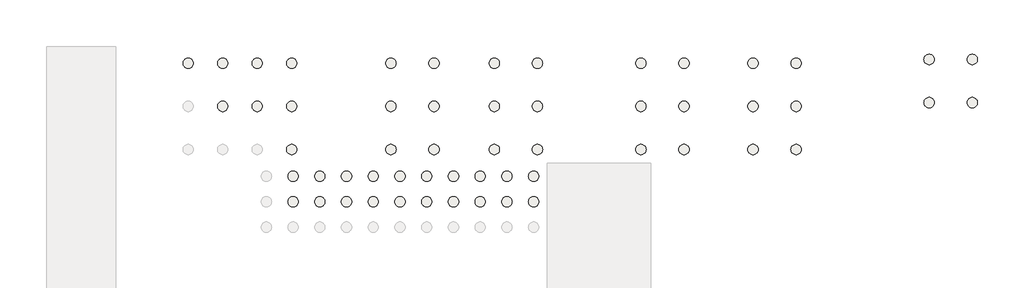
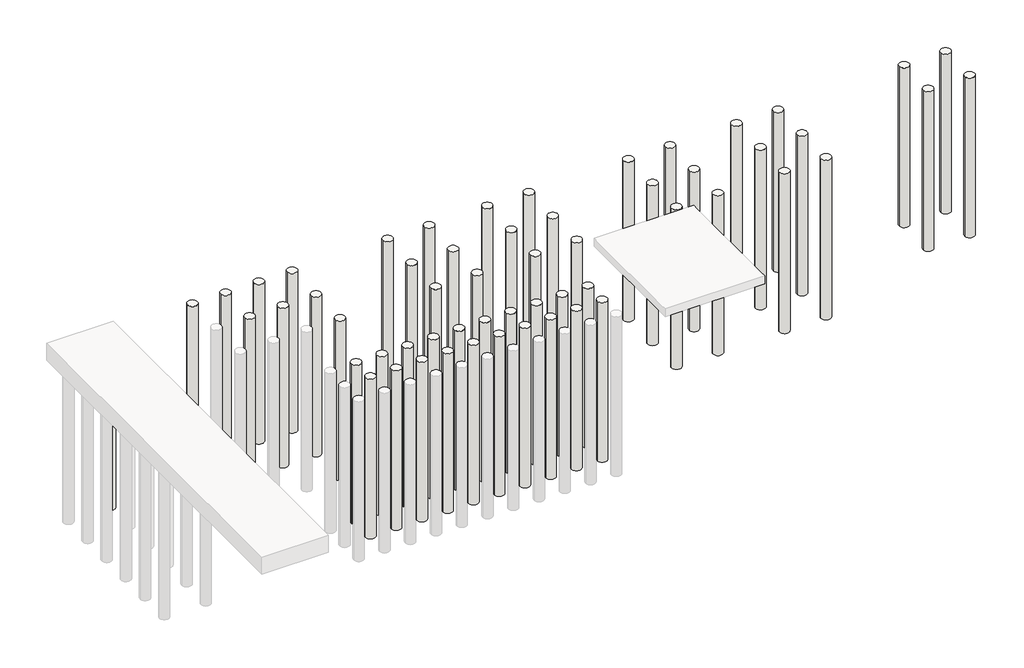
# One storey, part 3 of 3: 57 slabs.
"""IFC4 building model written with IfcOpenShell, lengths in millimetres."""

import ifcopenshell
import ifcopenshell.guid

model = None  # the IFC model being written
_history = None  # IfcOwnerHistory: only IFC2X3 demands one
_inside = {}  # id of a spatial element -> (the spatial element, [elements in it])
_under = {}  # id of a project, library or spatial element -> (it, [spatial elements below it])
_declared = {}  # id of a project -> (the project, [libraries it declares])
_typed = {}  # id of a type object -> (the type object, [elements of that type])
_made_of = {}  # id of a material, layer set ... -> (it, [elements and type objects made of it])


def new_model(schema):
    """Start an empty IFC model of exactly this schema.

    Asked for "IFC4X3", IfcOpenShell would pick the latest addendum, in which some entities
    have other attributes; the version numbers below select the first issue.
    IFC2X3 requires an IfcOwnerHistory on every rooted entity: one is made here for all.
    """
    global model, _history
    if schema == "IFC4X3":
        model = ifcopenshell.file(schema_version=(4, 3, 0, 0))
    else:
        model = ifcopenshell.file(schema=schema)
    _inside.clear()
    _under.clear()
    _declared.clear()
    _typed.clear()
    _made_of.clear()
    _history = None
    if model.schema == "IFC2X3":
        org = make("IfcOrganization", Name="unknown")
        user = make(
            "IfcPersonAndOrganization",
            ThePerson=make("IfcPerson", FamilyName="unknown"),
            TheOrganization=org,
        )
        app = make(
            "IfcApplication",
            ApplicationDeveloper=org,
            Version="unknown",
            ApplicationFullName="unknown",
            ApplicationIdentifier="unknown",
        )
        _history = make(
            "IfcOwnerHistory",
            OwningUser=user,
            OwningApplication=app,
            ChangeAction="ADDED",
            CreationDate=0,
        )
    return model


def make(cls, **values):
    """One entity of the class cls with the attributes given. An attribute that is None is left unset."""
    return model.create_entity(
        cls, **{name: value for name, value in values.items() if value is not None}
    )


def rooted(cls, **values):
    """An entity with a GlobalId (a new one), such as an element, a storey or a relation."""
    return make(cls, GlobalId=ifcopenshell.guid.new(), OwnerHistory=_history, **values)


def si_unit(unit_type, name, prefix=None):
    """IfcSIUnit, for example si_unit("LENGTHUNIT", "METRE", prefix="MILLI")."""
    return make("IfcSIUnit", UnitType=unit_type, Prefix=prefix, Name=name)


def assignment(units):
    """IfcUnitAssignment: the units of a project."""
    return None if units is None else make("IfcUnitAssignment", Units=units)


def point(xyz):
    """IfcCartesianPoint."""
    return None if xyz is None else make("IfcCartesianPoint", Coordinates=xyz)


def direction(xyz):
    """IfcDirection."""
    return None if xyz is None else make("IfcDirection", DirectionRatios=xyz)


def frame(location, z_axis=None, x_axis=None):
    """IfcAxis2Placement3D, a coordinate frame: its origin and axes. An axis left out is left unset."""
    return make(
        "IfcAxis2Placement3D",
        Location=point(location),
        Axis=direction(z_axis),
        RefDirection=direction(x_axis),
    )


def frame_2d(location, x_axis=None):
    """IfcAxis2Placement2D, a coordinate frame in the plane: its origin and x axis."""
    return make(
        "IfcAxis2Placement2D", Location=point(location), RefDirection=direction(x_axis)
    )


def origin():
    """The frame at (0, 0, 0) with its axes left unset."""
    return frame((0.0, 0.0, 0.0))


def place(relative_to, where):
    """IfcLocalPlacement: puts the frame where relative to a parent placement (None: the world)."""
    return make(
        "IfcLocalPlacement", PlacementRelTo=relative_to, RelativePlacement=where
    )


def context(
    kind, dimensions, precision=None, world=None, true_north=None, identifier=None
):
    """IfcGeometricRepresentationContext, for example the 3D "Model" context."""
    return make(
        "IfcGeometricRepresentationContext",
        ContextIdentifier=identifier,
        ContextType=kind,
        CoordinateSpaceDimension=dimensions,
        Precision=precision,
        WorldCoordinateSystem=world,
        TrueNorth=true_north,
    )


def project(units=None, contexts=None):
    """IfcProject with its units and contexts."""
    return rooted(
        "IfcProject",
        Name="project",
        RepresentationContexts=contexts,
        UnitsInContext=assignment(units),
    )


def spatial(cls, under=None, at=None, **own):
    """A site, building, storey or space (cls), placed at a placement, below another one or the project."""
    s = rooted(cls, ObjectPlacement=at, **own)
    if under is not None:
        _under.setdefault(under.id(), (under, []))[1].append(s)
    return s


def circle_curve(where, radius):
    """IfcCircle in the frame where."""
    return make("IfcCircle", Position=where, Radius=radius)


def trimmed(basis, trim1, trim2, sense, master):
    """IfcTrimmedCurve: the piece of a basis curve between two trims."""
    return make(
        "IfcTrimmedCurve",
        BasisCurve=basis,
        Trim1=trim1,
        Trim2=trim2,
        SenseAgreement=sense,
        MasterRepresentation=master,
    )


def segment(curve, same_sense, transition):
    """IfcCompositeCurveSegment."""
    return make(
        "IfcCompositeCurveSegment",
        Transition=transition,
        SameSense=same_sense,
        ParentCurve=curve,
    )


def composite_curve(segments, self_intersect=None):
    """IfcCompositeCurve: segments joined end to end."""
    return make("IfcCompositeCurve", Segments=segments, SelfIntersect=self_intersect)


def outline(outer, holes=None, kind="AREA"):
    """IfcArbitraryClosedProfileDef: a profile drawn as a closed curve; with holes, ...WithVoids."""
    if holes is None:
        return make("IfcArbitraryClosedProfileDef", ProfileType=kind, OuterCurve=outer)
    return make(
        "IfcArbitraryProfileDefWithVoids",
        ProfileType=kind,
        OuterCurve=outer,
        InnerCurves=holes,
    )


def extrude(swept, where, along, depth):
    """IfcExtrudedAreaSolid: the profile swept, set in the frame where, extruded along a direction by depth."""
    return make(
        "IfcExtrudedAreaSolid",
        SweptArea=swept,
        Position=where,
        ExtrudedDirection=direction(along),
        Depth=depth,
    )


def shape(context_of_items, identifier, shape_type, items):
    """IfcShapeRepresentation: the items that make up one representation, for example the "Body"."""
    return make(
        "IfcShapeRepresentation",
        ContextOfItems=context_of_items,
        RepresentationIdentifier=identifier,
        RepresentationType=shape_type,
        Items=items,
    )


def made_of(thing, what):
    """Note that an element or type object is made of a material, layer set ...; save() writes the relation."""
    if what is not None:
        _made_of.setdefault(what.id(), (what, []))[1].append(thing)
    return thing


def element(
    cls,
    number,
    at=None,
    inside=None,
    cuts=None,
    type_object=None,
    material=None,
    context=None,
    identifier="Body",
    shape_type=None,
    held_by="IfcProductDefinitionShape",
    body=None,
    shapes=None,
    **own,
):
    """One element of the class cls, such as IfcWall. Its Tag is "e" and its number.

    at: its placement. inside: the storey or other place that contains it. cuts: it is an
    opening in that element (IfcRelVoidsElement). A single representation is given by context,
    identifier, shape_type and body (its items); several are given by shapes. held_by: the class
    of the entity that holds the representations. save() writes the other relations.
    """
    e = rooted(cls, Tag="e%d" % number, ObjectPlacement=at, **own)
    if body is not None:
        shapes = [shape(context, identifier, shape_type, body)]
    if shapes is not None:
        e.Representation = make(held_by, Representations=shapes)
    if inside is not None:
        _inside.setdefault(inside.id(), (inside, []))[1].append(e)
    if cuts is not None:
        rooted(
            "IfcRelVoidsElement", RelatingBuildingElement=cuts, RelatedOpeningElement=e
        )
    if type_object is not None:
        _typed.setdefault(type_object.id(), (type_object, []))[1].append(e)
    return made_of(e, material)


def aggregate(whole, parts):
    """IfcRelAggregates: a whole, such as a stair, and the parts it consists of."""
    return rooted("IfcRelAggregates", RelatingObject=whole, RelatedObjects=parts)


def save(model, path):
    """Write the relations noted so far, then the file.

    IfcRelAggregates (storeys below a building ...), IfcRelContainedInSpatialStructure (elements
    in a storey), IfcRelDefinesByType, IfcRelAssociatesMaterial and IfcRelDeclares: one each for
    every whole, place, type object, material and project.
    """
    for whole, parts in _under.values():
        aggregate(whole, parts)
    for where, things in _inside.values():
        rooted(
            "IfcRelContainedInSpatialStructure",
            RelatedElements=things,
            RelatingStructure=where,
        )
    for kind, things in _typed.values():
        rooted("IfcRelDefinesByType", RelatedObjects=things, RelatingType=kind)
    for what, things in _made_of.values():
        rooted("IfcRelAssociatesMaterial", RelatedObjects=things, RelatingMaterial=what)
    for by, libraries in _declared.values():
        rooted("IfcRelDeclares", RelatingContext=by, RelatedDefinitions=libraries)
    model.write(path)


model = new_model("IFC4")

# Units and contexts
model_context = context("Model", 3, world=origin())
ifc_project = project(units=[si_unit("LENGTHUNIT", "METRE", prefix="MILLI")], contexts=[model_context])

# Site, building, storey
site = spatial("IfcSite", under=ifc_project)
building = spatial("IfcBuilding", under=site)
storey = spatial("IfcBuildingStorey", under=building, Name="B.O.F(FDN)", Elevation=-2500.0279945)

# Slabs
placement = place(None, origin())
element("IfcSlab", 1, ObjectType="Pile : H_SF_API_Steel Pile D508x12t_L10m", at=placement, inside=storey, context=model_context, shape_type="SweptSolid", body=[
    extrude(outline(composite_curve([segment(trimmed(circle_curve(frame_2d((1035.0, 40249.5208589)), 300.0), [point((1335.0, 40249.5208589))], [point((735.0, 40249.5208589))], False, "CARTESIAN"), True, "CONTINUOUS"), segment(trimmed(circle_curve(frame_2d((1035.0, 40249.5208589)), 300.0), [point((735.0, 40249.5208589))], [point((1335.0, 40249.5208589))], False, "CARTESIAN"), True, "CONTINUOUS")], self_intersect=False)), frame((0.0, 0.0, -13500.0279945), z_axis=(0.0, 0.0, 1.0), x_axis=(1.0, 0.0, 0.0)), (0.0, 0.0, 1.0), 10150.0),
])
element("IfcSlab", 2, ObjectType="Pile : H_SF_API_Steel Pile D508x12t_L10m", at=placement, inside=storey, context=model_context, shape_type="SweptSolid", body=[
    extrude(outline(composite_curve([segment(trimmed(circle_curve(frame_2d((51465.0, 37969.5208589)), 300.0), [point((51765.0, 37969.5208589))], [point((51165.0, 37969.5208589))], False, "CARTESIAN"), True, "CONTINUOUS"), segment(trimmed(circle_curve(frame_2d((51465.0, 37969.5208589)), 300.0), [point((51165.0, 37969.5208589))], [point((51765.0, 37969.5208589))], False, "CARTESIAN"), True, "CONTINUOUS")], self_intersect=False)), frame((0.0, 0.0, -12400.0279945), z_axis=(0.0, 0.0, 1.0), x_axis=(1.0, 0.0, 0.0)), (0.0, 0.0, 1.0), 10150.0),
])
element("IfcSlab", 3, ObjectType="Pile : H_SF_API_Steel Pile D508x12t_L10m", at=placement, inside=storey, context=model_context, shape_type="SweptSolid", body=[
    extrude(outline(composite_curve([segment(trimmed(circle_curve(frame_2d((48965.0, 37969.5208589)), 300.0), [point((48665.0, 37969.5208589))], [point((49265.0, 37969.5208589))], False, "CARTESIAN"), True, "CONTINUOUS"), segment(trimmed(circle_curve(frame_2d((48965.0, 37969.5208589)), 300.0), [point((49265.0, 37969.5208589))], [point((48665.0, 37969.5208589))], False, "CARTESIAN"), True, "CONTINUOUS")], self_intersect=False)), frame((0.0, 0.0, -12400.0279945), z_axis=(0.0, 0.0, 1.0), x_axis=(1.0, 0.0, 0.0)), (0.0, 0.0, 1.0), 10150.0),
])
element("IfcSlab", 4, ObjectType="Pile : H_SF_API_Steel Pile D508x12t_L10m", at=placement, inside=storey, context=model_context, shape_type="SweptSolid", body=[
    extrude(outline(composite_curve([segment(trimmed(circle_curve(frame_2d((51465.0, 40469.5208589)), 300.0), [point((51765.0, 40469.5208589))], [point((51165.0, 40469.5208589))], False, "CARTESIAN"), True, "CONTINUOUS"), segment(trimmed(circle_curve(frame_2d((51465.0, 40469.5208589)), 300.0), [point((51165.0, 40469.5208589))], [point((51765.0, 40469.5208589))], False, "CARTESIAN"), True, "CONTINUOUS")], self_intersect=False)), frame((0.0, 0.0, -12400.0279945), z_axis=(0.0, 0.0, 1.0), x_axis=(1.0, 0.0, 0.0)), (0.0, 0.0, 1.0), 10150.0),
])
element("IfcSlab", 5, ObjectType="Pile : H_SF_API_Steel Pile D508x12t_L10m", at=placement, inside=storey, context=model_context, shape_type="SweptSolid", body=[
    extrude(outline(composite_curve([segment(trimmed(circle_curve(frame_2d((48965.0, 40469.5208589)), 300.0), [point((48665.0, 40469.5208589))], [point((49265.0, 40469.5208589))], False, "CARTESIAN"), True, "CONTINUOUS"), segment(trimmed(circle_curve(frame_2d((48965.0, 40469.5208589)), 300.0), [point((49265.0, 40469.5208589))], [point((48665.0, 40469.5208589))], False, "CARTESIAN"), True, "CONTINUOUS")], self_intersect=False)), frame((0.0, 0.0, -12400.0279945), z_axis=(0.0, 0.0, 1.0), x_axis=(1.0, 0.0, 0.0)), (0.0, 0.0, 1.0), 10150.0),
])
element("IfcSlab", 6, ObjectType="Pile : H_SF_API_Steel Pile D508x12t_L10m", at=placement, inside=storey, context=model_context, shape_type="SweptSolid", body=[
    extrude(outline(composite_curve([segment(trimmed(circle_curve(frame_2d((6000.0, 40249.5208589)), 300.0), [point((5700.0, 40249.5208589))], [point((6300.0, 40249.5208589))], False, "CARTESIAN"), True, "CONTINUOUS"), segment(trimmed(circle_curve(frame_2d((6000.0, 40249.5208589)), 300.0), [point((6300.0, 40249.5208589))], [point((5700.0, 40249.5208589))], False, "CARTESIAN"), True, "CONTINUOUS")], self_intersect=False)), frame((0.0, 0.0, -12400.0279945), z_axis=(0.0, 0.0, 1.0), x_axis=(1.0, 0.0, 0.0)), (0.0, 0.0, 1.0), 10150.0),
])
element("IfcSlab", 7, ObjectType="Pile : H_SF_API_Steel Pile D508x12t_L10m", at=placement, inside=storey, context=model_context, shape_type="SweptSolid", body=[
    extrude(outline(composite_curve([segment(trimmed(circle_curve(frame_2d((8000.0, 40249.5208589)), 300.0), [point((8300.0, 40249.5208589))], [point((7700.0, 40249.5208589))], False, "CARTESIAN"), True, "CONTINUOUS"), segment(trimmed(circle_curve(frame_2d((8000.0, 40249.5208589)), 300.0), [point((7700.0, 40249.5208589))], [point((8300.0, 40249.5208589))], False, "CARTESIAN"), True, "CONTINUOUS")], self_intersect=False)), frame((0.0, 0.0, -12400.0279945), z_axis=(0.0, 0.0, 1.0), x_axis=(1.0, 0.0, 0.0)), (0.0, 0.0, 1.0), 10150.0),
])
element("IfcSlab", 8, ObjectType="Pile : H_SF_API_Steel Pile D508x12t_L10m", at=placement, inside=storey, context=model_context, shape_type="SweptSolid", body=[
    extrude(outline(composite_curve([segment(trimmed(circle_curve(frame_2d((8000.0, 37749.5208589)), 300.0), [point((8300.0, 37749.5208589))], [point((7700.0, 37749.5208589))], False, "CARTESIAN"), True, "CONTINUOUS"), segment(trimmed(circle_curve(frame_2d((8000.0, 37749.5208589)), 300.0), [point((7700.0, 37749.5208589))], [point((8300.0, 37749.5208589))], False, "CARTESIAN"), True, "CONTINUOUS")], self_intersect=False)), frame((0.0, 0.0, -12400.0279945), z_axis=(0.0, 0.0, 1.0), x_axis=(1.0, 0.0, 0.0)), (0.0, 0.0, 1.0), 10150.0),
])
element("IfcSlab", 9, ObjectType="Pile : H_SF_API_Steel Pile D508x12t_L10m", at=placement, inside=storey, context=model_context, shape_type="SweptSolid", body=[
    extrude(outline(composite_curve([segment(trimmed(circle_curve(frame_2d((10000.0, 40249.5208589)), 300.0), [point((9700.0, 40249.5208589))], [point((10300.0, 40249.5208589))], False, "CARTESIAN"), True, "CONTINUOUS"), segment(trimmed(circle_curve(frame_2d((10000.0, 40249.5208589)), 300.0), [point((10300.0, 40249.5208589))], [point((9700.0, 40249.5208589))], False, "CARTESIAN"), True, "CONTINUOUS")], self_intersect=False)), frame((0.0, 0.0, -12400.0279945), z_axis=(0.0, 0.0, 1.0), x_axis=(1.0, 0.0, 0.0)), (0.0, 0.0, 1.0), 10150.0),
])
element("IfcSlab", 10, ObjectType="Pile : H_SF_API_Steel Pile D508x12t_L10m", at=placement, inside=storey, context=model_context, shape_type="SweptSolid", body=[
    extrude(outline(composite_curve([segment(trimmed(circle_curve(frame_2d((12000.0, 40249.5208589)), 300.0), [point((12300.0, 40249.5208589))], [point((11700.0, 40249.5208589))], False, "CARTESIAN"), True, "CONTINUOUS"), segment(trimmed(circle_curve(frame_2d((12000.0, 40249.5208589)), 300.0), [point((11700.0, 40249.5208589))], [point((12300.0, 40249.5208589))], False, "CARTESIAN"), True, "CONTINUOUS")], self_intersect=False)), frame((0.0, 0.0, -12400.0279945), z_axis=(0.0, 0.0, 1.0), x_axis=(1.0, 0.0, 0.0)), (0.0, 0.0, 1.0), 10150.0),
])
element("IfcSlab", 11, ObjectType="Pile : H_SF_API_Steel Pile D508x12t_L10m", at=placement, inside=storey, context=model_context, shape_type="SweptSolid", body=[
    extrude(outline(composite_curve([segment(trimmed(circle_curve(frame_2d((10000.0, 37749.5208589)), 300.0), [point((9700.0, 37749.5208589))], [point((10300.0, 37749.5208589))], False, "CARTESIAN"), True, "CONTINUOUS"), segment(trimmed(circle_curve(frame_2d((10000.0, 37749.5208589)), 300.0), [point((10300.0, 37749.5208589))], [point((9700.0, 37749.5208589))], False, "CARTESIAN"), True, "CONTINUOUS")], self_intersect=False)), frame((0.0, 0.0, -12400.0279945), z_axis=(0.0, 0.0, 1.0), x_axis=(1.0, 0.0, 0.0)), (0.0, 0.0, 1.0), 10150.0),
])
element("IfcSlab", 12, ObjectType="Pile : H_SF_API_Steel Pile D508x12t_L10m", at=placement, inside=storey, context=model_context, shape_type="SweptSolid", body=[
    extrude(outline(composite_curve([segment(trimmed(circle_curve(frame_2d((12000.0, 37749.5208589)), 300.0), [point((12300.0, 37749.5208589))], [point((11700.0, 37749.5208589))], False, "CARTESIAN"), True, "CONTINUOUS"), segment(trimmed(circle_curve(frame_2d((12000.0, 37749.5208589)), 300.0), [point((11700.0, 37749.5208589))], [point((12300.0, 37749.5208589))], False, "CARTESIAN"), True, "CONTINUOUS")], self_intersect=False)), frame((0.0, 0.0, -12400.0279945), z_axis=(0.0, 0.0, 1.0), x_axis=(1.0, 0.0, 0.0)), (0.0, 0.0, 1.0), 10150.0),
])
element("IfcSlab", 13, ObjectType="Pile : H_SF_API_Steel Pile D508x12t_L10m", at=placement, inside=storey, context=model_context, shape_type="SweptSolid", body=[
    extrude(outline(composite_curve([segment(trimmed(circle_curve(frame_2d((12000.0, 35249.5208589)), 300.0), [point((12300.0, 35249.5208589))], [point((11700.0, 35249.5208589))], False, "CARTESIAN"), True, "CONTINUOUS"), segment(trimmed(circle_curve(frame_2d((12000.0, 35249.5208589)), 300.0), [point((11700.0, 35249.5208589))], [point((12300.0, 35249.5208589))], False, "CARTESIAN"), True, "CONTINUOUS")], self_intersect=False)), frame((0.0, 0.0, -12400.0279945), z_axis=(0.0, 0.0, 1.0), x_axis=(1.0, 0.0, 0.0)), (0.0, 0.0, 1.0), 10150.0),
])
element("IfcSlab", 14, ObjectType="Pile : H_SF_API_Steel Pile D508x12t_L10m", at=placement, inside=storey, context=model_context, shape_type="SweptSolid", body=[
    extrude(outline(composite_curve([segment(trimmed(circle_curve(frame_2d((20250.0, 40249.5208589)), 300.0), [point((20550.0, 40249.5208589))], [point((19950.0, 40249.5208589))], False, "CARTESIAN"), True, "CONTINUOUS"), segment(trimmed(circle_curve(frame_2d((20250.0, 40249.5208589)), 300.0), [point((19950.0, 40249.5208589))], [point((20550.0, 40249.5208589))], False, "CARTESIAN"), True, "CONTINUOUS")], self_intersect=False)), frame((0.0, 0.0, -12400.0279945), z_axis=(0.0, 0.0, 1.0), x_axis=(1.0, 0.0, 0.0)), (0.0, 0.0, 1.0), 10150.0),
])
element("IfcSlab", 15, ObjectType="Pile : H_SF_API_Steel Pile D508x12t_L10m", at=placement, inside=storey, context=model_context, shape_type="SweptSolid", body=[
    extrude(outline(composite_curve([segment(trimmed(circle_curve(frame_2d((17750.0, 40249.5208589)), 300.0), [point((17450.0, 40249.5208589))], [point((18050.0, 40249.5208589))], False, "CARTESIAN"), True, "CONTINUOUS"), segment(trimmed(circle_curve(frame_2d((17750.0, 40249.5208589)), 300.0), [point((18050.0, 40249.5208589))], [point((17450.0, 40249.5208589))], False, "CARTESIAN"), True, "CONTINUOUS")], self_intersect=False)), frame((0.0, 0.0, -12400.0279945), z_axis=(0.0, 0.0, 1.0), x_axis=(1.0, 0.0, 0.0)), (0.0, 0.0, 1.0), 10150.0),
])
element("IfcSlab", 16, ObjectType="Pile : H_SF_API_Steel Pile D508x12t_L10m", at=placement, inside=storey, context=model_context, shape_type="SweptSolid", body=[
    extrude(outline(composite_curve([segment(trimmed(circle_curve(frame_2d((20250.0, 37749.5208589)), 300.0), [point((20550.0, 37749.5208589))], [point((19950.0, 37749.5208589))], False, "CARTESIAN"), True, "CONTINUOUS"), segment(trimmed(circle_curve(frame_2d((20250.0, 37749.5208589)), 300.0), [point((19950.0, 37749.5208589))], [point((20550.0, 37749.5208589))], False, "CARTESIAN"), True, "CONTINUOUS")], self_intersect=False)), frame((0.0, 0.0, -12400.0279945), z_axis=(0.0, 0.0, 1.0), x_axis=(1.0, 0.0, 0.0)), (0.0, 0.0, 1.0), 10150.0),
])
element("IfcSlab", 17, ObjectType="Pile : H_SF_API_Steel Pile D508x12t_L10m", at=placement, inside=storey, context=model_context, shape_type="SweptSolid", body=[
    extrude(outline(composite_curve([segment(trimmed(circle_curve(frame_2d((17750.0, 37749.5208589)), 300.0), [point((17450.0, 37749.5208589))], [point((18050.0, 37749.5208589))], False, "CARTESIAN"), True, "CONTINUOUS"), segment(trimmed(circle_curve(frame_2d((17750.0, 37749.5208589)), 300.0), [point((18050.0, 37749.5208589))], [point((17450.0, 37749.5208589))], False, "CARTESIAN"), True, "CONTINUOUS")], self_intersect=False)), frame((0.0, 0.0, -12400.0279945), z_axis=(0.0, 0.0, 1.0), x_axis=(1.0, 0.0, 0.0)), (0.0, 0.0, 1.0), 10150.0),
])
element("IfcSlab", 18, ObjectType="Pile : H_SF_API_Steel Pile D508x12t_L10m", at=placement, inside=storey, context=model_context, shape_type="SweptSolid", body=[
    extrude(outline(composite_curve([segment(trimmed(circle_curve(frame_2d((20250.0, 35249.5208589)), 300.0), [point((20550.0, 35249.5208589))], [point((19950.0, 35249.5208589))], False, "CARTESIAN"), True, "CONTINUOUS"), segment(trimmed(circle_curve(frame_2d((20250.0, 35249.5208589)), 300.0), [point((19950.0, 35249.5208589))], [point((20550.0, 35249.5208589))], False, "CARTESIAN"), True, "CONTINUOUS")], self_intersect=False)), frame((0.0, 0.0, -12400.0279945), z_axis=(0.0, 0.0, 1.0), x_axis=(1.0, 0.0, 0.0)), (0.0, 0.0, 1.0), 10150.0),
])
element("IfcSlab", 19, ObjectType="Pile : H_SF_API_Steel Pile D508x12t_L10m", at=placement, inside=storey, context=model_context, shape_type="SweptSolid", body=[
    extrude(outline(composite_curve([segment(trimmed(circle_curve(frame_2d((17750.0, 35249.5208589)), 300.0), [point((17450.0, 35249.5208589))], [point((18050.0, 35249.5208589))], False, "CARTESIAN"), True, "CONTINUOUS"), segment(trimmed(circle_curve(frame_2d((17750.0, 35249.5208589)), 300.0), [point((18050.0, 35249.5208589))], [point((17450.0, 35249.5208589))], False, "CARTESIAN"), True, "CONTINUOUS")], self_intersect=False)), frame((0.0, 0.0, -12400.0279945), z_axis=(0.0, 0.0, 1.0), x_axis=(1.0, 0.0, 0.0)), (0.0, 0.0, 1.0), 10150.0),
])
element("IfcSlab", 20, ObjectType="Pile : H_SF_API_Steel Pile D508x12t_L10m", at=placement, inside=storey, context=model_context, shape_type="SweptSolid", body=[
    extrude(outline(composite_curve([segment(trimmed(circle_curve(frame_2d((26250.0, 40249.5208589)), 300.0), [point((26550.0, 40249.5208589))], [point((25950.0, 40249.5208589))], False, "CARTESIAN"), True, "CONTINUOUS"), segment(trimmed(circle_curve(frame_2d((26250.0, 40249.5208589)), 300.0), [point((25950.0, 40249.5208589))], [point((26550.0, 40249.5208589))], False, "CARTESIAN"), True, "CONTINUOUS")], self_intersect=False)), frame((0.0, 0.0, -12400.0279945), z_axis=(0.0, 0.0, 1.0), x_axis=(1.0, 0.0, 0.0)), (0.0, 0.0, 1.0), 10150.0),
])
element("IfcSlab", 21, ObjectType="Pile : H_SF_API_Steel Pile D508x12t_L10m", at=placement, inside=storey, context=model_context, shape_type="SweptSolid", body=[
    extrude(outline(composite_curve([segment(trimmed(circle_curve(frame_2d((23750.0, 40249.5208589)), 300.0), [point((23450.0, 40249.5208589))], [point((24050.0, 40249.5208589))], False, "CARTESIAN"), True, "CONTINUOUS"), segment(trimmed(circle_curve(frame_2d((23750.0, 40249.5208589)), 300.0), [point((24050.0, 40249.5208589))], [point((23450.0, 40249.5208589))], False, "CARTESIAN"), True, "CONTINUOUS")], self_intersect=False)), frame((0.0, 0.0, -12400.0279945), z_axis=(0.0, 0.0, 1.0), x_axis=(1.0, 0.0, 0.0)), (0.0, 0.0, 1.0), 10150.0),
])
element("IfcSlab", 22, ObjectType="Pile : H_SF_API_Steel Pile D508x12t_L10m", at=placement, inside=storey, context=model_context, shape_type="SweptSolid", body=[
    extrude(outline(composite_curve([segment(trimmed(circle_curve(frame_2d((26250.0, 37749.5208589)), 300.0), [point((26550.0, 37749.5208589))], [point((25950.0, 37749.5208589))], False, "CARTESIAN"), True, "CONTINUOUS"), segment(trimmed(circle_curve(frame_2d((26250.0, 37749.5208589)), 300.0), [point((25950.0, 37749.5208589))], [point((26550.0, 37749.5208589))], False, "CARTESIAN"), True, "CONTINUOUS")], self_intersect=False)), frame((0.0, 0.0, -12400.0279945), z_axis=(0.0, 0.0, 1.0), x_axis=(1.0, 0.0, 0.0)), (0.0, 0.0, 1.0), 10150.0),
])
element("IfcSlab", 23, ObjectType="Pile : H_SF_API_Steel Pile D508x12t_L10m", at=placement, inside=storey, context=model_context, shape_type="SweptSolid", body=[
    extrude(outline(composite_curve([segment(trimmed(circle_curve(frame_2d((23750.0, 37749.5208589)), 300.0), [point((23450.0, 37749.5208589))], [point((24050.0, 37749.5208589))], False, "CARTESIAN"), True, "CONTINUOUS"), segment(trimmed(circle_curve(frame_2d((23750.0, 37749.5208589)), 300.0), [point((24050.0, 37749.5208589))], [point((23450.0, 37749.5208589))], False, "CARTESIAN"), True, "CONTINUOUS")], self_intersect=False)), frame((0.0, 0.0, -12400.0279945), z_axis=(0.0, 0.0, 1.0), x_axis=(1.0, 0.0, 0.0)), (0.0, 0.0, 1.0), 10150.0),
])
element("IfcSlab", 24, ObjectType="Pile : H_SF_API_Steel Pile D508x12t_L10m", at=placement, inside=storey, context=model_context, shape_type="SweptSolid", body=[
    extrude(outline(composite_curve([segment(trimmed(circle_curve(frame_2d((26250.0, 35249.5208589)), 300.0), [point((26550.0, 35249.5208589))], [point((25950.0, 35249.5208589))], False, "CARTESIAN"), True, "CONTINUOUS"), segment(trimmed(circle_curve(frame_2d((26250.0, 35249.5208589)), 300.0), [point((25950.0, 35249.5208589))], [point((26550.0, 35249.5208589))], False, "CARTESIAN"), True, "CONTINUOUS")], self_intersect=False)), frame((0.0, 0.0, -12400.0279945), z_axis=(0.0, 0.0, 1.0), x_axis=(1.0, 0.0, 0.0)), (0.0, 0.0, 1.0), 10150.0),
])
element("IfcSlab", 25, ObjectType="Pile : H_SF_API_Steel Pile D508x12t_L10m", at=placement, inside=storey, context=model_context, shape_type="SweptSolid", body=[
    extrude(outline(composite_curve([segment(trimmed(circle_curve(frame_2d((23750.0, 35249.5208589)), 300.0), [point((23450.0, 35249.5208589))], [point((24050.0, 35249.5208589))], False, "CARTESIAN"), True, "CONTINUOUS"), segment(trimmed(circle_curve(frame_2d((23750.0, 35249.5208589)), 300.0), [point((24050.0, 35249.5208589))], [point((23450.0, 35249.5208589))], False, "CARTESIAN"), True, "CONTINUOUS")], self_intersect=False)), frame((0.0, 0.0, -12400.0279945), z_axis=(0.0, 0.0, 1.0), x_axis=(1.0, 0.0, 0.0)), (0.0, 0.0, 1.0), 10150.0),
])
element("IfcSlab", 26, ObjectType="Pile : H_SF_API_Steel Pile D508x12t_L10m", at=placement, inside=storey, context=model_context, shape_type="SweptSolid", body=[
    extrude(outline(composite_curve([segment(trimmed(circle_curve(frame_2d((34750.0, 40249.5208589)), 300.0), [point((35050.0, 40249.5208589))], [point((34450.0, 40249.5208589))], False, "CARTESIAN"), True, "CONTINUOUS"), segment(trimmed(circle_curve(frame_2d((34750.0, 40249.5208589)), 300.0), [point((34450.0, 40249.5208589))], [point((35050.0, 40249.5208589))], False, "CARTESIAN"), True, "CONTINUOUS")], self_intersect=False)), frame((0.0, 0.0, -12400.0279945), z_axis=(0.0, 0.0, 1.0), x_axis=(1.0, 0.0, 0.0)), (0.0, 0.0, 1.0), 10150.0),
])
element("IfcSlab", 27, ObjectType="Pile : H_SF_API_Steel Pile D508x12t_L10m", at=placement, inside=storey, context=model_context, shape_type="SweptSolid", body=[
    extrude(outline(composite_curve([segment(trimmed(circle_curve(frame_2d((32250.0, 40249.5208589)), 300.0), [point((31950.0, 40249.5208589))], [point((32550.0, 40249.5208589))], False, "CARTESIAN"), True, "CONTINUOUS"), segment(trimmed(circle_curve(frame_2d((32250.0, 40249.5208589)), 300.0), [point((32550.0, 40249.5208589))], [point((31950.0, 40249.5208589))], False, "CARTESIAN"), True, "CONTINUOUS")], self_intersect=False)), frame((0.0, 0.0, -12400.0279945), z_axis=(0.0, 0.0, 1.0), x_axis=(1.0, 0.0, 0.0)), (0.0, 0.0, 1.0), 10150.0),
])
element("IfcSlab", 28, ObjectType="Pile : H_SF_API_Steel Pile D508x12t_L10m", at=placement, inside=storey, context=model_context, shape_type="SweptSolid", body=[
    extrude(outline(composite_curve([segment(trimmed(circle_curve(frame_2d((34750.0, 37749.5208589)), 300.0), [point((35050.0, 37749.5208589))], [point((34450.0, 37749.5208589))], False, "CARTESIAN"), True, "CONTINUOUS"), segment(trimmed(circle_curve(frame_2d((34750.0, 37749.5208589)), 300.0), [point((34450.0, 37749.5208589))], [point((35050.0, 37749.5208589))], False, "CARTESIAN"), True, "CONTINUOUS")], self_intersect=False)), frame((0.0, 0.0, -12400.0279945), z_axis=(0.0, 0.0, 1.0), x_axis=(1.0, 0.0, 0.0)), (0.0, 0.0, 1.0), 10150.0),
])
element("IfcSlab", 29, ObjectType="Pile : H_SF_API_Steel Pile D508x12t_L10m", at=placement, inside=storey, context=model_context, shape_type="SweptSolid", body=[
    extrude(outline(composite_curve([segment(trimmed(circle_curve(frame_2d((32250.0, 37749.5208589)), 300.0), [point((31950.0, 37749.5208589))], [point((32550.0, 37749.5208589))], False, "CARTESIAN"), True, "CONTINUOUS"), segment(trimmed(circle_curve(frame_2d((32250.0, 37749.5208589)), 300.0), [point((32550.0, 37749.5208589))], [point((31950.0, 37749.5208589))], False, "CARTESIAN"), True, "CONTINUOUS")], self_intersect=False)), frame((0.0, 0.0, -12400.0279945), z_axis=(0.0, 0.0, 1.0), x_axis=(1.0, 0.0, 0.0)), (0.0, 0.0, 1.0), 10150.0),
])
element("IfcSlab", 30, ObjectType="Pile : H_SF_API_Steel Pile D508x12t_L10m", at=placement, inside=storey, context=model_context, shape_type="SweptSolid", body=[
    extrude(outline(composite_curve([segment(trimmed(circle_curve(frame_2d((34750.0, 35249.5208589)), 300.0), [point((35050.0, 35249.5208589))], [point((34450.0, 35249.5208589))], False, "CARTESIAN"), True, "CONTINUOUS"), segment(trimmed(circle_curve(frame_2d((34750.0, 35249.5208589)), 300.0), [point((34450.0, 35249.5208589))], [point((35050.0, 35249.5208589))], False, "CARTESIAN"), True, "CONTINUOUS")], self_intersect=False)), frame((0.0, 0.0, -12400.0279945), z_axis=(0.0, 0.0, 1.0), x_axis=(1.0, 0.0, 0.0)), (0.0, 0.0, 1.0), 10150.0),
])
element("IfcSlab", 31, ObjectType="Pile : H_SF_API_Steel Pile D508x12t_L10m", at=placement, inside=storey, context=model_context, shape_type="SweptSolid", body=[
    extrude(outline(composite_curve([segment(trimmed(circle_curve(frame_2d((32250.0, 35249.5208589)), 300.0), [point((31950.0, 35249.5208589))], [point((32550.0, 35249.5208589))], False, "CARTESIAN"), True, "CONTINUOUS"), segment(trimmed(circle_curve(frame_2d((32250.0, 35249.5208589)), 300.0), [point((32550.0, 35249.5208589))], [point((31950.0, 35249.5208589))], False, "CARTESIAN"), True, "CONTINUOUS")], self_intersect=False)), frame((0.0, 0.0, -12400.0279945), z_axis=(0.0, 0.0, 1.0), x_axis=(1.0, 0.0, 0.0)), (0.0, 0.0, 1.0), 10150.0),
])
element("IfcSlab", 32, ObjectType="Pile : H_SF_API_Steel Pile D508x12t_L10m", at=placement, inside=storey, context=model_context, shape_type="SweptSolid", body=[
    extrude(outline(composite_curve([segment(trimmed(circle_curve(frame_2d((41250.0, 40249.5208589)), 300.0), [point((41550.0, 40249.5208589))], [point((40950.0, 40249.5208589))], False, "CARTESIAN"), True, "CONTINUOUS"), segment(trimmed(circle_curve(frame_2d((41250.0, 40249.5208589)), 300.0), [point((40950.0, 40249.5208589))], [point((41550.0, 40249.5208589))], False, "CARTESIAN"), True, "CONTINUOUS")], self_intersect=False)), frame((0.0, 0.0, -12400.0279945), z_axis=(0.0, 0.0, 1.0), x_axis=(1.0, 0.0, 0.0)), (0.0, 0.0, 1.0), 10150.0),
])
element("IfcSlab", 33, ObjectType="Pile : H_SF_API_Steel Pile D508x12t_L10m", at=placement, inside=storey, context=model_context, shape_type="SweptSolid", body=[
    extrude(outline(composite_curve([segment(trimmed(circle_curve(frame_2d((38750.0, 40249.5208589)), 300.0), [point((38450.0, 40249.5208589))], [point((39050.0, 40249.5208589))], False, "CARTESIAN"), True, "CONTINUOUS"), segment(trimmed(circle_curve(frame_2d((38750.0, 40249.5208589)), 300.0), [point((39050.0, 40249.5208589))], [point((38450.0, 40249.5208589))], False, "CARTESIAN"), True, "CONTINUOUS")], self_intersect=False)), frame((0.0, 0.0, -12400.0279945), z_axis=(0.0, 0.0, 1.0), x_axis=(1.0, 0.0, 0.0)), (0.0, 0.0, 1.0), 10150.0),
])
element("IfcSlab", 34, ObjectType="Pile : H_SF_API_Steel Pile D508x12t_L10m", at=placement, inside=storey, context=model_context, shape_type="SweptSolid", body=[
    extrude(outline(composite_curve([segment(trimmed(circle_curve(frame_2d((41250.0, 37749.5208589)), 300.0), [point((41550.0, 37749.5208589))], [point((40950.0, 37749.5208589))], False, "CARTESIAN"), True, "CONTINUOUS"), segment(trimmed(circle_curve(frame_2d((41250.0, 37749.5208589)), 300.0), [point((40950.0, 37749.5208589))], [point((41550.0, 37749.5208589))], False, "CARTESIAN"), True, "CONTINUOUS")], self_intersect=False)), frame((0.0, 0.0, -12400.0279945), z_axis=(0.0, 0.0, 1.0), x_axis=(1.0, 0.0, 0.0)), (0.0, 0.0, 1.0), 10150.0),
])
element("IfcSlab", 35, ObjectType="Pile : H_SF_API_Steel Pile D508x12t_L10m", at=placement, inside=storey, context=model_context, shape_type="SweptSolid", body=[
    extrude(outline(composite_curve([segment(trimmed(circle_curve(frame_2d((38750.0, 37749.5208589)), 300.0), [point((38450.0, 37749.5208589))], [point((39050.0, 37749.5208589))], False, "CARTESIAN"), True, "CONTINUOUS"), segment(trimmed(circle_curve(frame_2d((38750.0, 37749.5208589)), 300.0), [point((39050.0, 37749.5208589))], [point((38450.0, 37749.5208589))], False, "CARTESIAN"), True, "CONTINUOUS")], self_intersect=False)), frame((0.0, 0.0, -12400.0279945), z_axis=(0.0, 0.0, 1.0), x_axis=(1.0, 0.0, 0.0)), (0.0, 0.0, 1.0), 10150.0),
])
element("IfcSlab", 36, ObjectType="Pile : H_SF_API_Steel Pile D508x12t_L10m", at=placement, inside=storey, context=model_context, shape_type="SweptSolid", body=[
    extrude(outline(composite_curve([segment(trimmed(circle_curve(frame_2d((41250.0, 35249.5208589)), 300.0), [point((41550.0, 35249.5208589))], [point((40950.0, 35249.5208589))], False, "CARTESIAN"), True, "CONTINUOUS"), segment(trimmed(circle_curve(frame_2d((41250.0, 35249.5208589)), 300.0), [point((40950.0, 35249.5208589))], [point((41550.0, 35249.5208589))], False, "CARTESIAN"), True, "CONTINUOUS")], self_intersect=False)), frame((0.0, 0.0, -12400.0279945), z_axis=(0.0, 0.0, 1.0), x_axis=(1.0, 0.0, 0.0)), (0.0, 0.0, 1.0), 10150.0),
])
element("IfcSlab", 37, ObjectType="Pile : H_SF_API_Steel Pile D508x12t_L10m", at=placement, inside=storey, context=model_context, shape_type="SweptSolid", body=[
    extrude(outline(composite_curve([segment(trimmed(circle_curve(frame_2d((38750.0, 35249.5208589)), 300.0), [point((38450.0, 35249.5208589))], [point((39050.0, 35249.5208589))], False, "CARTESIAN"), True, "CONTINUOUS"), segment(trimmed(circle_curve(frame_2d((38750.0, 35249.5208589)), 300.0), [point((39050.0, 35249.5208589))], [point((38450.0, 35249.5208589))], False, "CARTESIAN"), True, "CONTINUOUS")], self_intersect=False)), frame((0.0, 0.0, -12400.0279945), z_axis=(0.0, 0.0, 1.0), x_axis=(1.0, 0.0, 0.0)), (0.0, 0.0, 1.0), 10150.0),
])
element("IfcSlab", 38, ObjectType="Pile : H_SF_API_Steel Pile D508x12t_L10m", at=placement, inside=storey, context=model_context, shape_type="SweptSolid", body=[
    extrude(outline(composite_curve([segment(trimmed(circle_curve(frame_2d((26030.0, 33699.5208589)), 300.0), [point((26330.0, 33699.5208589))], [point((25730.0, 33699.5208589))], False, "CARTESIAN"), True, "CONTINUOUS"), segment(trimmed(circle_curve(frame_2d((26030.0, 33699.5208589)), 300.0), [point((25730.0, 33699.5208589))], [point((26330.0, 33699.5208589))], False, "CARTESIAN"), True, "CONTINUOUS")], self_intersect=False)), frame((0.0, 0.0, -14300.0279945), z_axis=(0.0, 0.0, 1.0), x_axis=(1.0, 0.0, 0.0)), (0.0, 0.0, 1.0), 10150.0),
])
element("IfcSlab", 39, ObjectType="Pile : H_SF_API_Steel Pile D508x12t_L10m", at=placement, inside=storey, context=model_context, shape_type="SweptSolid", body=[
    extrude(outline(composite_curve([segment(trimmed(circle_curve(frame_2d((26030.0, 32224.5208589)), 300.0), [point((26330.0, 32224.5208589))], [point((25730.0, 32224.5208589))], False, "CARTESIAN"), True, "CONTINUOUS"), segment(trimmed(circle_curve(frame_2d((26030.0, 32224.5208589)), 300.0), [point((25730.0, 32224.5208589))], [point((26330.0, 32224.5208589))], False, "CARTESIAN"), True, "CONTINUOUS")], self_intersect=False)), frame((0.0, 0.0, -14300.0279945), z_axis=(0.0, 0.0, 1.0), x_axis=(1.0, 0.0, 0.0)), (0.0, 0.0, 1.0), 10150.0),
])
element("IfcSlab", 40, ObjectType="Pile : H_SF_API_Steel Pile D508x12t_L10m", at=placement, inside=storey, context=model_context, shape_type="SweptSolid", body=[
    extrude(outline(composite_curve([segment(trimmed(circle_curve(frame_2d((24480.0, 33699.5208589)), 300.0), [point((24780.0, 33699.5208589))], [point((24180.0, 33699.5208589))], False, "CARTESIAN"), True, "CONTINUOUS"), segment(trimmed(circle_curve(frame_2d((24480.0, 33699.5208589)), 300.0), [point((24180.0, 33699.5208589))], [point((24780.0, 33699.5208589))], False, "CARTESIAN"), True, "CONTINUOUS")], self_intersect=False)), frame((0.0, 0.0, -14300.0279945), z_axis=(0.0, 0.0, 1.0), x_axis=(1.0, 0.0, 0.0)), (0.0, 0.0, 1.0), 10150.0),
])
element("IfcSlab", 41, ObjectType="Pile : H_SF_API_Steel Pile D508x12t_L10m", at=placement, inside=storey, context=model_context, shape_type="SweptSolid", body=[
    extrude(outline(composite_curve([segment(trimmed(circle_curve(frame_2d((24480.0, 32224.5208589)), 300.0), [point((24780.0, 32224.5208589))], [point((24180.0, 32224.5208589))], False, "CARTESIAN"), True, "CONTINUOUS"), segment(trimmed(circle_curve(frame_2d((24480.0, 32224.5208589)), 300.0), [point((24180.0, 32224.5208589))], [point((24780.0, 32224.5208589))], False, "CARTESIAN"), True, "CONTINUOUS")], self_intersect=False)), frame((0.0, 0.0, -14300.0279945), z_axis=(0.0, 0.0, 1.0), x_axis=(1.0, 0.0, 0.0)), (0.0, 0.0, 1.0), 10150.0),
])
element("IfcSlab", 42, ObjectType="Pile : H_SF_API_Steel Pile D508x12t_L10m", at=placement, inside=storey, context=model_context, shape_type="SweptSolid", body=[
    extrude(outline(composite_curve([segment(trimmed(circle_curve(frame_2d((22930.0, 33699.5208589)), 300.0), [point((23230.0, 33699.5208589))], [point((22630.0, 33699.5208589))], False, "CARTESIAN"), True, "CONTINUOUS"), segment(trimmed(circle_curve(frame_2d((22930.0, 33699.5208589)), 300.0), [point((22630.0, 33699.5208589))], [point((23230.0, 33699.5208589))], False, "CARTESIAN"), True, "CONTINUOUS")], self_intersect=False)), frame((0.0, 0.0, -14300.0279945), z_axis=(0.0, 0.0, 1.0), x_axis=(1.0, 0.0, 0.0)), (0.0, 0.0, 1.0), 10150.0),
])
element("IfcSlab", 43, ObjectType="Pile : H_SF_API_Steel Pile D508x12t_L10m", at=placement, inside=storey, context=model_context, shape_type="SweptSolid", body=[
    extrude(outline(composite_curve([segment(trimmed(circle_curve(frame_2d((22930.0, 32224.5208589)), 300.0), [point((23230.0, 32224.5208589))], [point((22630.0, 32224.5208589))], False, "CARTESIAN"), True, "CONTINUOUS"), segment(trimmed(circle_curve(frame_2d((22930.0, 32224.5208589)), 300.0), [point((22630.0, 32224.5208589))], [point((23230.0, 32224.5208589))], False, "CARTESIAN"), True, "CONTINUOUS")], self_intersect=False)), frame((0.0, 0.0, -14300.0279945), z_axis=(0.0, 0.0, 1.0), x_axis=(1.0, 0.0, 0.0)), (0.0, 0.0, 1.0), 10150.0),
])
element("IfcSlab", 44, ObjectType="Pile : H_SF_API_Steel Pile D508x12t_L10m", at=placement, inside=storey, context=model_context, shape_type="SweptSolid", body=[
    extrude(outline(composite_curve([segment(trimmed(circle_curve(frame_2d((21380.0, 33699.5208589)), 300.0), [point((21680.0, 33699.5208589))], [point((21080.0, 33699.5208589))], False, "CARTESIAN"), True, "CONTINUOUS"), segment(trimmed(circle_curve(frame_2d((21380.0, 33699.5208589)), 300.0), [point((21080.0, 33699.5208589))], [point((21680.0, 33699.5208589))], False, "CARTESIAN"), True, "CONTINUOUS")], self_intersect=False)), frame((0.0, 0.0, -14300.0279945), z_axis=(0.0, 0.0, 1.0), x_axis=(1.0, 0.0, 0.0)), (0.0, 0.0, 1.0), 10150.0),
])
element("IfcSlab", 45, ObjectType="Pile : H_SF_API_Steel Pile D508x12t_L10m", at=placement, inside=storey, context=model_context, shape_type="SweptSolid", body=[
    extrude(outline(composite_curve([segment(trimmed(circle_curve(frame_2d((21380.0, 32224.5208589)), 300.0), [point((21680.0, 32224.5208589))], [point((21080.0, 32224.5208589))], False, "CARTESIAN"), True, "CONTINUOUS"), segment(trimmed(circle_curve(frame_2d((21380.0, 32224.5208589)), 300.0), [point((21080.0, 32224.5208589))], [point((21680.0, 32224.5208589))], False, "CARTESIAN"), True, "CONTINUOUS")], self_intersect=False)), frame((0.0, 0.0, -14300.0279945), z_axis=(0.0, 0.0, 1.0), x_axis=(1.0, 0.0, 0.0)), (0.0, 0.0, 1.0), 10150.0),
])
element("IfcSlab", 46, ObjectType="Pile : H_SF_API_Steel Pile D508x12t_L10m", at=placement, inside=storey, context=model_context, shape_type="SweptSolid", body=[
    extrude(outline(composite_curve([segment(trimmed(circle_curve(frame_2d((19830.0, 33699.5208589)), 300.0), [point((20130.0, 33699.5208589))], [point((19530.0, 33699.5208589))], False, "CARTESIAN"), True, "CONTINUOUS"), segment(trimmed(circle_curve(frame_2d((19830.0, 33699.5208589)), 300.0), [point((19530.0, 33699.5208589))], [point((20130.0, 33699.5208589))], False, "CARTESIAN"), True, "CONTINUOUS")], self_intersect=False)), frame((0.0, 0.0, -14300.0279945), z_axis=(0.0, 0.0, 1.0), x_axis=(1.0, 0.0, 0.0)), (0.0, 0.0, 1.0), 10150.0),
])
element("IfcSlab", 47, ObjectType="Pile : H_SF_API_Steel Pile D508x12t_L10m", at=placement, inside=storey, context=model_context, shape_type="SweptSolid", body=[
    extrude(outline(composite_curve([segment(trimmed(circle_curve(frame_2d((19830.0, 32224.5208589)), 300.0), [point((20130.0, 32224.5208589))], [point((19530.0, 32224.5208589))], False, "CARTESIAN"), True, "CONTINUOUS"), segment(trimmed(circle_curve(frame_2d((19830.0, 32224.5208589)), 300.0), [point((19530.0, 32224.5208589))], [point((20130.0, 32224.5208589))], False, "CARTESIAN"), True, "CONTINUOUS")], self_intersect=False)), frame((0.0, 0.0, -14300.0279945), z_axis=(0.0, 0.0, 1.0), x_axis=(1.0, 0.0, 0.0)), (0.0, 0.0, 1.0), 10150.0),
])
element("IfcSlab", 48, ObjectType="Pile : H_SF_API_Steel Pile D508x12t_L10m", at=placement, inside=storey, context=model_context, shape_type="SweptSolid", body=[
    extrude(outline(composite_curve([segment(trimmed(circle_curve(frame_2d((18280.0, 33699.5208589)), 300.0), [point((18580.0, 33699.5208589))], [point((17980.0, 33699.5208589))], False, "CARTESIAN"), True, "CONTINUOUS"), segment(trimmed(circle_curve(frame_2d((18280.0, 33699.5208589)), 300.0), [point((17980.0, 33699.5208589))], [point((18580.0, 33699.5208589))], False, "CARTESIAN"), True, "CONTINUOUS")], self_intersect=False)), frame((0.0, 0.0, -14300.0279945), z_axis=(0.0, 0.0, 1.0), x_axis=(1.0, 0.0, 0.0)), (0.0, 0.0, 1.0), 10150.0),
])
element("IfcSlab", 49, ObjectType="Pile : H_SF_API_Steel Pile D508x12t_L10m", at=placement, inside=storey, context=model_context, shape_type="SweptSolid", body=[
    extrude(outline(composite_curve([segment(trimmed(circle_curve(frame_2d((18280.0, 32224.5208589)), 300.0), [point((18580.0, 32224.5208589))], [point((17980.0, 32224.5208589))], False, "CARTESIAN"), True, "CONTINUOUS"), segment(trimmed(circle_curve(frame_2d((18280.0, 32224.5208589)), 300.0), [point((17980.0, 32224.5208589))], [point((18580.0, 32224.5208589))], False, "CARTESIAN"), True, "CONTINUOUS")], self_intersect=False)), frame((0.0, 0.0, -14300.0279945), z_axis=(0.0, 0.0, 1.0), x_axis=(1.0, 0.0, 0.0)), (0.0, 0.0, 1.0), 10150.0),
])
element("IfcSlab", 50, ObjectType="Pile : H_SF_API_Steel Pile D508x12t_L10m", at=placement, inside=storey, context=model_context, shape_type="SweptSolid", body=[
    extrude(outline(composite_curve([segment(trimmed(circle_curve(frame_2d((16730.0, 33699.5208589)), 300.0), [point((17030.0, 33699.5208589))], [point((16430.0, 33699.5208589))], False, "CARTESIAN"), True, "CONTINUOUS"), segment(trimmed(circle_curve(frame_2d((16730.0, 33699.5208589)), 300.0), [point((16430.0, 33699.5208589))], [point((17030.0, 33699.5208589))], False, "CARTESIAN"), True, "CONTINUOUS")], self_intersect=False)), frame((0.0, 0.0, -14300.0279945), z_axis=(0.0, 0.0, 1.0), x_axis=(1.0, 0.0, 0.0)), (0.0, 0.0, 1.0), 10150.0),
])
element("IfcSlab", 51, ObjectType="Pile : H_SF_API_Steel Pile D508x12t_L10m", at=placement, inside=storey, context=model_context, shape_type="SweptSolid", body=[
    extrude(outline(composite_curve([segment(trimmed(circle_curve(frame_2d((16730.0, 32224.5208589)), 300.0), [point((17030.0, 32224.5208589))], [point((16430.0, 32224.5208589))], False, "CARTESIAN"), True, "CONTINUOUS"), segment(trimmed(circle_curve(frame_2d((16730.0, 32224.5208589)), 300.0), [point((16430.0, 32224.5208589))], [point((17030.0, 32224.5208589))], False, "CARTESIAN"), True, "CONTINUOUS")], self_intersect=False)), frame((0.0, 0.0, -14300.0279945), z_axis=(0.0, 0.0, 1.0), x_axis=(1.0, 0.0, 0.0)), (0.0, 0.0, 1.0), 10150.0),
])
element("IfcSlab", 52, ObjectType="Pile : H_SF_API_Steel Pile D508x12t_L10m", at=placement, inside=storey, context=model_context, shape_type="SweptSolid", body=[
    extrude(outline(composite_curve([segment(trimmed(circle_curve(frame_2d((15180.0, 33699.5208589)), 300.0), [point((15480.0, 33699.5208589))], [point((14880.0, 33699.5208589))], False, "CARTESIAN"), True, "CONTINUOUS"), segment(trimmed(circle_curve(frame_2d((15180.0, 33699.5208589)), 300.0), [point((14880.0, 33699.5208589))], [point((15480.0, 33699.5208589))], False, "CARTESIAN"), True, "CONTINUOUS")], self_intersect=False)), frame((0.0, 0.0, -14300.0279945), z_axis=(0.0, 0.0, 1.0), x_axis=(1.0, 0.0, 0.0)), (0.0, 0.0, 1.0), 10150.0),
])
element("IfcSlab", 53, ObjectType="Pile : H_SF_API_Steel Pile D508x12t_L10m", at=placement, inside=storey, context=model_context, shape_type="SweptSolid", body=[
    extrude(outline(composite_curve([segment(trimmed(circle_curve(frame_2d((15180.0, 32224.5208589)), 300.0), [point((15480.0, 32224.5208589))], [point((14880.0, 32224.5208589))], False, "CARTESIAN"), True, "CONTINUOUS"), segment(trimmed(circle_curve(frame_2d((15180.0, 32224.5208589)), 300.0), [point((14880.0, 32224.5208589))], [point((15480.0, 32224.5208589))], False, "CARTESIAN"), True, "CONTINUOUS")], self_intersect=False)), frame((0.0, 0.0, -14300.0279945), z_axis=(0.0, 0.0, 1.0), x_axis=(1.0, 0.0, 0.0)), (0.0, 0.0, 1.0), 10150.0),
])
element("IfcSlab", 54, ObjectType="Pile : H_SF_API_Steel Pile D508x12t_L10m", at=placement, inside=storey, context=model_context, shape_type="SweptSolid", body=[
    extrude(outline(composite_curve([segment(trimmed(circle_curve(frame_2d((13630.0, 33699.5208589)), 300.0), [point((13930.0, 33699.5208589))], [point((13330.0, 33699.5208589))], False, "CARTESIAN"), True, "CONTINUOUS"), segment(trimmed(circle_curve(frame_2d((13630.0, 33699.5208589)), 300.0), [point((13330.0, 33699.5208589))], [point((13930.0, 33699.5208589))], False, "CARTESIAN"), True, "CONTINUOUS")], self_intersect=False)), frame((0.0, 0.0, -14300.0279945), z_axis=(0.0, 0.0, 1.0), x_axis=(1.0, 0.0, 0.0)), (0.0, 0.0, 1.0), 10150.0),
])
element("IfcSlab", 55, ObjectType="Pile : H_SF_API_Steel Pile D508x12t_L10m", at=placement, inside=storey, context=model_context, shape_type="SweptSolid", body=[
    extrude(outline(composite_curve([segment(trimmed(circle_curve(frame_2d((13630.0, 32224.5208589)), 300.0), [point((13930.0, 32224.5208589))], [point((13330.0, 32224.5208589))], False, "CARTESIAN"), True, "CONTINUOUS"), segment(trimmed(circle_curve(frame_2d((13630.0, 32224.5208589)), 300.0), [point((13330.0, 32224.5208589))], [point((13930.0, 32224.5208589))], False, "CARTESIAN"), True, "CONTINUOUS")], self_intersect=False)), frame((0.0, 0.0, -14300.0279945), z_axis=(0.0, 0.0, 1.0), x_axis=(1.0, 0.0, 0.0)), (0.0, 0.0, 1.0), 10150.0),
])
element("IfcSlab", 56, ObjectType="Pile : H_SF_API_Steel Pile D508x12t_L10m", at=placement, inside=storey, context=model_context, shape_type="SweptSolid", body=[
    extrude(outline(composite_curve([segment(trimmed(circle_curve(frame_2d((12080.0, 33699.5208589)), 300.0), [point((12380.0, 33699.5208589))], [point((11780.0, 33699.5208589))], False, "CARTESIAN"), True, "CONTINUOUS"), segment(trimmed(circle_curve(frame_2d((12080.0, 33699.5208589)), 300.0), [point((11780.0, 33699.5208589))], [point((12380.0, 33699.5208589))], False, "CARTESIAN"), True, "CONTINUOUS")], self_intersect=False)), frame((0.0, 0.0, -14300.0279945), z_axis=(0.0, 0.0, 1.0), x_axis=(1.0, 0.0, 0.0)), (0.0, 0.0, 1.0), 10150.0),
])
element("IfcSlab", 57, ObjectType="Pile : H_SF_API_Steel Pile D508x12t_L10m", at=placement, inside=storey, context=model_context, shape_type="SweptSolid", body=[
    extrude(outline(composite_curve([segment(trimmed(circle_curve(frame_2d((12080.0, 32224.5208589)), 300.0), [point((12380.0, 32224.5208589))], [point((11780.0, 32224.5208589))], False, "CARTESIAN"), True, "CONTINUOUS"), segment(trimmed(circle_curve(frame_2d((12080.0, 32224.5208589)), 300.0), [point((11780.0, 32224.5208589))], [point((12380.0, 32224.5208589))], False, "CARTESIAN"), True, "CONTINUOUS")], self_intersect=False)), frame((0.0, 0.0, -14300.0279945), z_axis=(0.0, 0.0, 1.0), x_axis=(1.0, 0.0, 0.0)), (0.0, 0.0, 1.0), 10150.0),
])

save(model, "model.ifc")

# Revit data of these elements
# Type "Pile : H_SF_API_Steel Pile D508x12t_L10m"
#   Assembly Code = "A1020130"
#   반지름 = 0.3000 m
#   최소 내포 = 0.1500 m
#   Diameter = 0.6000 m
#   Depth = 10.0000 m
#   VISIBLE [instance default] = yes
#   구조 재료 = 콘크리트
# Elements 1, 2, 3, 4, 5, 6, 7, 8, 9, 10, 11, 12, 13, 14, 15, 16, 17, 18, 19, 21, 23, 25, 26, 27, 28, 29, 30, 31, 32, 33, 34, 35, 36, 37, 42, 43, 44, 45, 46, 47, 48, 49, 50, 51, 52, 53, 54, 55, 56, 57 (IfcSlab, "Pile : H_SF_API_Steel Pile D508x12t_L10m")
#   Phase Created = New Construction
#   Materials on its faces: "금속 - 스틸 - 345MPa"
# Elements 20, 22, 24, 38, 39, 40, 41 (IfcSlab, "Pile : H_SF_API_Steel Pile D508x12t_L10m")
#   VISIBLE = yes
#   Phase Created = New Construction
#   Materials on its faces: "금속 - 스틸 - 345MPa"
# Materials
#   "콘크리트": class "*D 철근콘크리트공사", colour RGB 192 192 192, transparency 0, Keynote = "DF", Description = "콘크리트", Cost = 0
#   "금속 - 스틸 - 345MPa": class "금속", colour RGB 247 247 247, transparency 0
